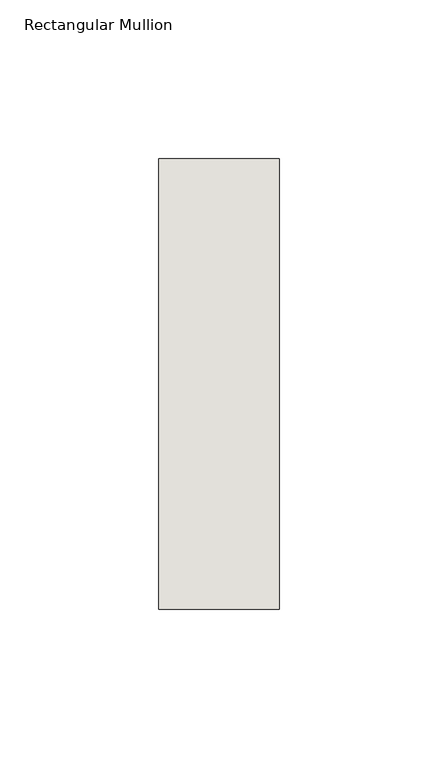
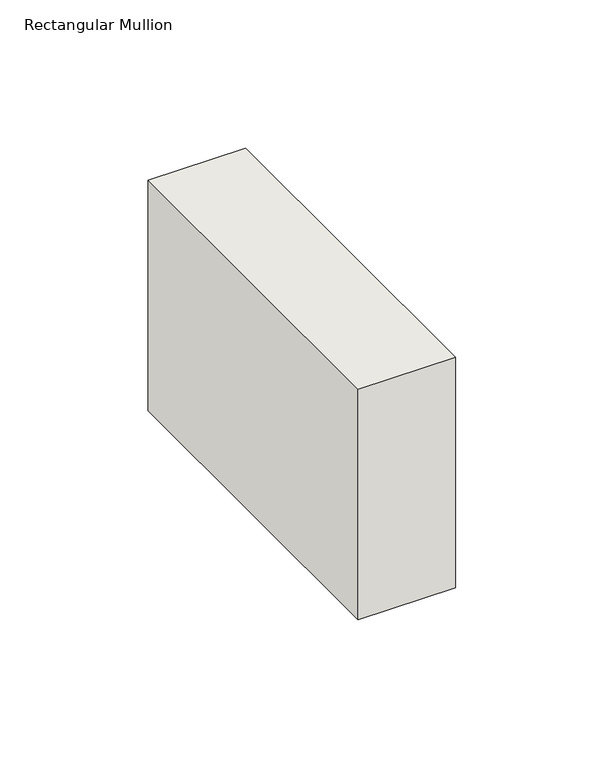
"""IFC4 building model written with IfcOpenShell, lengths in millimetres: wall geometry, Rectangular Mullion : NLRS_21_CWM_hsb-regel 38x142_gen_rsf."""

from ifc_helpers import new_model, si_unit, frame, origin, place, context, project, spatial, polyline, outline, extrude, source, transform, mapped, element, save


def rectangular_mullion_3dbdc851(model_context):
    return source(origin(), model_context, "Body", "SweptSolid", [
        extrude(outline(polyline([(-38.0, -71.0), (-38.0, 71.0), (0.0, 71.0), (0.0, -71.0), (-38.0, -71.0)])), frame((0.0, 0.0, -94.9999997), z_axis=(0.0, 0.0, 1.0), x_axis=(1.0, 0.0, 0.0)), (0.0, 0.0, 1.0), 94.9999997),
    ])


if __name__ == "__main__":
    model = new_model("IFC4")
    model_context = context("Model", 3, world=origin())
    ifc_project = project(units=[si_unit("LENGTHUNIT", "METRE", prefix="MILLI")], contexts=[model_context])
    site = spatial("IfcSite", under=ifc_project)
    building = spatial("IfcBuilding", under=site)
    placement = place(None, origin())
    rectangular_mullion_shape = rectangular_mullion_3dbdc851(model_context)
    element("IfcWall", 1, ObjectType="Rectangular Mullion : NLRS_21_CWM_hsb-regel 38x142_gen_rsf", at=placement, inside=building, context=model_context, shape_type="MappedRepresentation", body=[
        mapped(rectangular_mullion_shape, transform((0.0, 0.0, 0.0), x_axis=(1.0, 0.0, 0.0), y_axis=(0.0, 1.0, 0.0), z_axis=(0.0, 0.0, 1.0))),
    ])
    save(model, "model.ifc")

# Revit data of these elements
# Type "Rectangular Mullion : NLRS_21_CWM_hsb-regel 38x142_gen_rsf"
#   Type IfcGUID = "07M7mRoiH1CR8m_RSKIwpF"
#   Assembly Code = "21.10"
#   IfcExportAs = "IfcWall"
#   built-in parameter 1007322 = 0.465879 (stored number, unit not read)
#   built-in parameter 1007321 = 0.062336 (stored number, unit not read)
#   built-in parameter 1007320 = 0.062336 (stored number, unit not read)
# Element 1 (IfcWall, "Rectangular Mullion : NLRS_21_CWM_hsb-regel 38x142_gen_rsf")
#   Materials on its faces: "NLRS_i2_hout naaldhout vuren_gen_rsf"
# Materials
#   "NLRS_i2_hout naaldhout vuren_gen_rsf": class "I - Hout", colour RGB 234 199 147, transparency 0, Keynote = "i2", Manufacturer = "Revit Standards Foundation", URL = "www.revitstandards.org", Description = "hout vuren", Cost = 0
